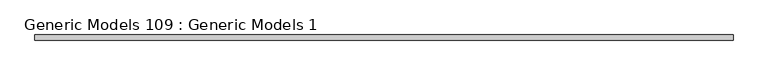
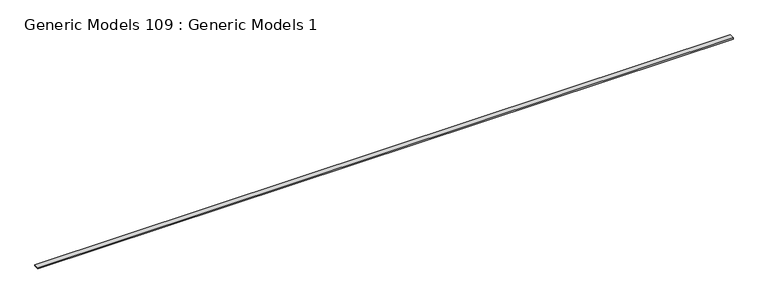
"""IFC4 building model written with IfcOpenShell, lengths in millimetres: proxy geometry, Generic Models 109 : Generic Models 1."""

from ifc_helpers import new_model, si_unit, frame, origin, place, context, project, spatial, polyline, outline, extrude, source, transform, mapped, element, save


def generic_models_109_generic_models_1_7cfb6ed3(model_context):
    return source(origin(), model_context, "Body", "SweptSolid", [
        extrude(outline(polyline([(-20998.9733045, 51294.7476718), (-20998.9733045, 51434.4476718), (-1948.9733045, 51434.4476718), (-1948.9733045, 51294.7476718), (-20998.9733045, 51294.7476718)])), frame((0.0, 0.0, 127066.3735933), z_axis=(0.0, 0.0, 1.0), x_axis=(1.0, 0.0, 0.0)), (0.0, 0.0, 1.0), 38.1),
    ])


if __name__ == "__main__":
    model = new_model("IFC4")
    model_context = context("Model", 3, world=origin())
    ifc_project = project(units=[si_unit("LENGTHUNIT", "METRE", prefix="MILLI")], contexts=[model_context])
    site = spatial("IfcSite", under=ifc_project)
    building = spatial("IfcBuilding", under=site)
    placement = place(None, origin())
    generic_models_109_generic_models_1_shape = generic_models_109_generic_models_1_7cfb6ed3(model_context)
    element("IfcBuildingElementProxy", 1, Name="Generic Models 109 : Generic Models 1", ObjectType="Generic Models 109 : Generic Models 1", at=placement, inside=building, context=model_context, shape_type="MappedRepresentation", body=[
        mapped(generic_models_109_generic_models_1_shape, transform((0.0, 0.0, 0.0), x_axis=(1.0, 0.0, 0.0), y_axis=(0.0, 1.0, 0.0), z_axis=(0.0, 0.0, 1.0))),
    ])
    save(model, "model.ifc")

# Revit data of these elements
# Element 1 (IfcBuildingElementProxy, "Generic Models 109 : Generic Models 1")
#   Materials on its faces: "_2X BLOCKING AS REQUIRED"
# Materials
#   "_2X BLOCKING AS REQUIRED": class "Generic", colour RGB 177 130 114, transparency 0, Cost = 0
